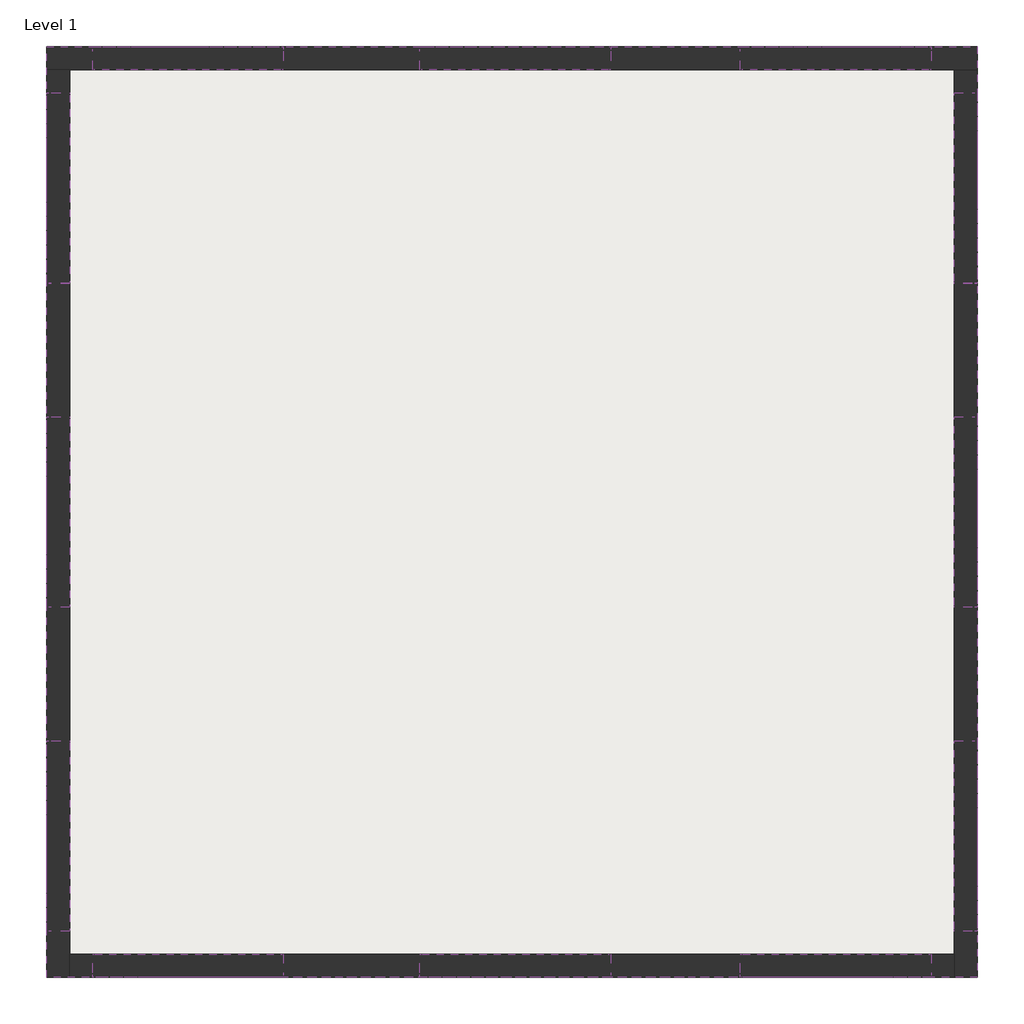
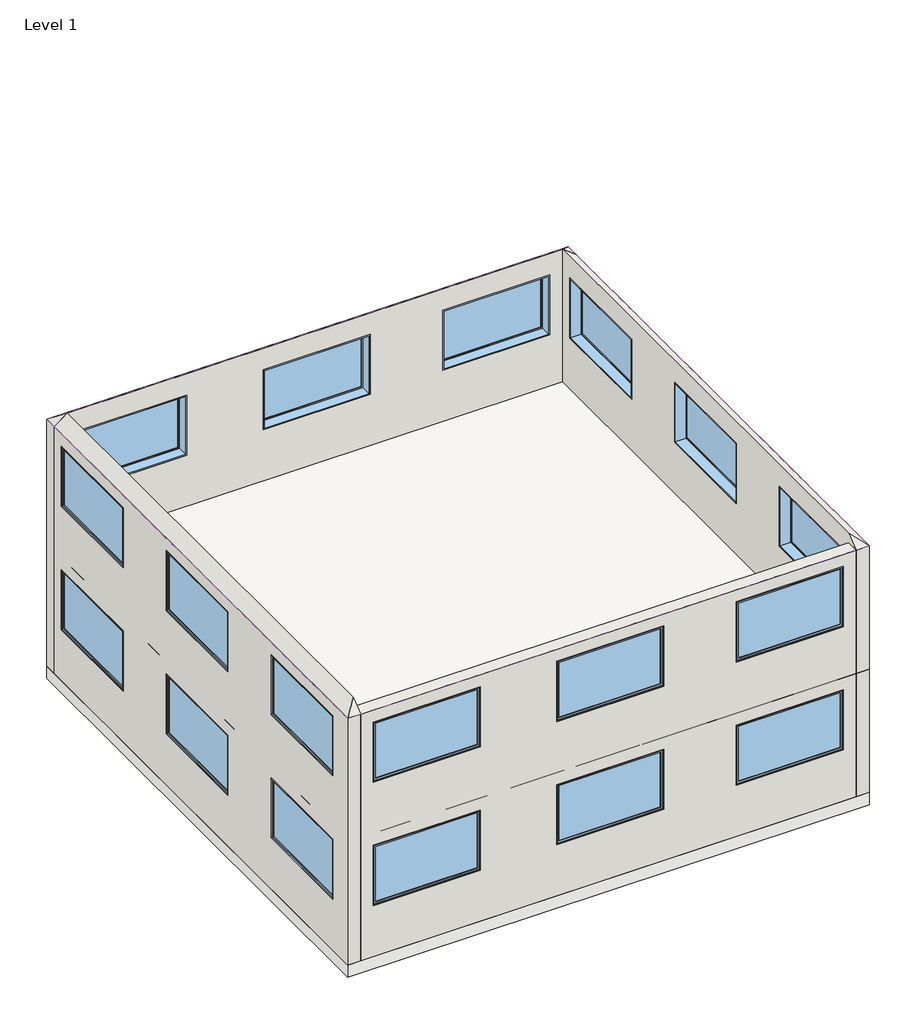
# One storey: 24 windows, 4 walls, 2 slabs, 1 roof.
"""IFC4 building model written with IfcOpenShell, lengths in millimetres."""

import ifcopenshell
import ifcopenshell.guid

model = None  # the IFC model being written
_history = None  # IfcOwnerHistory: only IFC2X3 demands one
_inside = {}  # id of a spatial element -> (the spatial element, [elements in it])
_under = {}  # id of a project, library or spatial element -> (it, [spatial elements below it])
_declared = {}  # id of a project -> (the project, [libraries it declares])
_typed = {}  # id of a type object -> (the type object, [elements of that type])
_made_of = {}  # id of a material, layer set ... -> (it, [elements and type objects made of it])


def new_model(schema):
    """Start an empty IFC model of exactly this schema.

    Asked for "IFC4X3", IfcOpenShell would pick the latest addendum, in which some entities
    have other attributes; the version numbers below select the first issue.
    IFC2X3 requires an IfcOwnerHistory on every rooted entity: one is made here for all.
    """
    global model, _history
    if schema == "IFC4X3":
        model = ifcopenshell.file(schema_version=(4, 3, 0, 0))
    else:
        model = ifcopenshell.file(schema=schema)
    _inside.clear()
    _under.clear()
    _declared.clear()
    _typed.clear()
    _made_of.clear()
    _history = None
    if model.schema == "IFC2X3":
        org = make("IfcOrganization", Name="unknown")
        user = make(
            "IfcPersonAndOrganization",
            ThePerson=make("IfcPerson", FamilyName="unknown"),
            TheOrganization=org,
        )
        app = make(
            "IfcApplication",
            ApplicationDeveloper=org,
            Version="unknown",
            ApplicationFullName="unknown",
            ApplicationIdentifier="unknown",
        )
        _history = make(
            "IfcOwnerHistory",
            OwningUser=user,
            OwningApplication=app,
            ChangeAction="ADDED",
            CreationDate=0,
        )
    return model


def make(cls, **values):
    """One entity of the class cls with the attributes given. An attribute that is None is left unset."""
    return model.create_entity(
        cls, **{name: value for name, value in values.items() if value is not None}
    )


def rooted(cls, **values):
    """An entity with a GlobalId (a new one), such as an element, a storey or a relation."""
    return make(cls, GlobalId=ifcopenshell.guid.new(), OwnerHistory=_history, **values)


def si_unit(unit_type, name, prefix=None):
    """IfcSIUnit, for example si_unit("LENGTHUNIT", "METRE", prefix="MILLI")."""
    return make("IfcSIUnit", UnitType=unit_type, Prefix=prefix, Name=name)


def assignment(units):
    """IfcUnitAssignment: the units of a project."""
    return None if units is None else make("IfcUnitAssignment", Units=units)


def point(xyz):
    """IfcCartesianPoint."""
    return None if xyz is None else make("IfcCartesianPoint", Coordinates=xyz)


def direction(xyz):
    """IfcDirection."""
    return None if xyz is None else make("IfcDirection", DirectionRatios=xyz)


def frame(location, z_axis=None, x_axis=None):
    """IfcAxis2Placement3D, a coordinate frame: its origin and axes. An axis left out is left unset."""
    return make(
        "IfcAxis2Placement3D",
        Location=point(location),
        Axis=direction(z_axis),
        RefDirection=direction(x_axis),
    )


def origin():
    """The frame at (0, 0, 0) with its axes left unset."""
    return frame((0.0, 0.0, 0.0))


def place(relative_to, where):
    """IfcLocalPlacement: puts the frame where relative to a parent placement (None: the world)."""
    return make(
        "IfcLocalPlacement", PlacementRelTo=relative_to, RelativePlacement=where
    )


def context(
    kind, dimensions, precision=None, world=None, true_north=None, identifier=None
):
    """IfcGeometricRepresentationContext, for example the 3D "Model" context."""
    return make(
        "IfcGeometricRepresentationContext",
        ContextIdentifier=identifier,
        ContextType=kind,
        CoordinateSpaceDimension=dimensions,
        Precision=precision,
        WorldCoordinateSystem=world,
        TrueNorth=true_north,
    )


def project(units=None, contexts=None):
    """IfcProject with its units and contexts."""
    return rooted(
        "IfcProject",
        Name="project",
        RepresentationContexts=contexts,
        UnitsInContext=assignment(units),
    )


def spatial(cls, under=None, at=None, **own):
    """A site, building, storey or space (cls), placed at a placement, below another one or the project."""
    s = rooted(cls, ObjectPlacement=at, **own)
    if under is not None:
        _under.setdefault(under.id(), (under, []))[1].append(s)
    return s


def polyline(points):
    """IfcPolyline through the points."""
    return make("IfcPolyline", Points=[point(p) for p in points])


def outline(outer, holes=None, kind="AREA"):
    """IfcArbitraryClosedProfileDef: a profile drawn as a closed curve; with holes, ...WithVoids."""
    if holes is None:
        return make("IfcArbitraryClosedProfileDef", ProfileType=kind, OuterCurve=outer)
    return make(
        "IfcArbitraryProfileDefWithVoids",
        ProfileType=kind,
        OuterCurve=outer,
        InnerCurves=holes,
    )


def extrude(swept, where, along, depth):
    """IfcExtrudedAreaSolid: the profile swept, set in the frame where, extruded along a direction by depth."""
    return make(
        "IfcExtrudedAreaSolid",
        SweptArea=swept,
        Position=where,
        ExtrudedDirection=direction(along),
        Depth=depth,
    )


def faces_of(points, faces, orient=None, outer=None):
    """IfcFace entities. A face is a list of loops; a loop is a list of indices into points, from 0.

    orient and outer hold one flag for each loop. By default every Orientation is true, the
    first loop of a face is its IfcFaceOuterBound and the others are IfcFaceBound.
    """
    made = []
    for i, loops in enumerate(faces):
        bounds = []
        for j, loop in enumerate(loops):
            is_outer = j == 0 if outer is None else outer[i][j]
            bounds.append(
                make(
                    "IfcFaceOuterBound" if is_outer else "IfcFaceBound",
                    Bound=make("IfcPolyLoop", Polygon=[points[k] for k in loop]),
                    Orientation=True if orient is None else orient[i][j],
                )
            )
        made.append(make("IfcFace", Bounds=bounds))
    return made


def faceted_brep(points, faces, orient=None, outer=None, voids=None):
    """IfcFacetedBrep: a solid bounded by flat faces; with voids (closed shells), ...WithVoids."""
    shared = [point(p) for p in points]
    hull = make("IfcClosedShell", CfsFaces=faces_of(shared, faces, orient, outer))
    if voids is None:
        return make("IfcFacetedBrep", Outer=hull)
    return make(
        "IfcFacetedBrepWithVoids",
        Outer=hull,
        Voids=[
            make(cls, CfsFaces=faces_of(shared, fs, o, b)) for cls, fs, o, b in voids
        ],
    )


def shape(context_of_items, identifier, shape_type, items):
    """IfcShapeRepresentation: the items that make up one representation, for example the "Body"."""
    return make(
        "IfcShapeRepresentation",
        ContextOfItems=context_of_items,
        RepresentationIdentifier=identifier,
        RepresentationType=shape_type,
        Items=items,
    )


def source(mapping_origin, context_of_items, identifier, shape_type, items):
    """IfcRepresentationMap: a shape defined once, which mapped items show again and again."""
    return make(
        "IfcRepresentationMap",
        MappingOrigin=mapping_origin,
        MappedRepresentation=shape(context_of_items, identifier, shape_type, items),
    )


def transform(
    local_origin,
    x_axis=None,
    y_axis=None,
    z_axis=None,
    scale=None,
    scale2=None,
    scale3=None,
    uniform=True,
):
    """IfcCartesianTransformationOperator3D, or its non-uniform kind. x_axis, y_axis, z_axis: its Axis1, 2, 3."""
    if uniform:
        return make(
            "IfcCartesianTransformationOperator3D",
            Axis1=direction(x_axis),
            Axis2=direction(y_axis),
            LocalOrigin=point(local_origin),
            Scale=scale,
            Axis3=direction(z_axis),
        )
    return make(
        "IfcCartesianTransformationOperator3DnonUniform",
        Axis1=direction(x_axis),
        Axis2=direction(y_axis),
        LocalOrigin=point(local_origin),
        Scale=scale,
        Axis3=direction(z_axis),
        Scale2=scale2,
        Scale3=scale3,
    )


def mapped(mapping_source, mapping_target):
    """IfcMappedItem: shows the shape of a source again, moved by a transform."""
    return make(
        "IfcMappedItem", MappingSource=mapping_source, MappingTarget=mapping_target
    )


def made_of(thing, what):
    """Note that an element or type object is made of a material, layer set ...; save() writes the relation."""
    if what is not None:
        _made_of.setdefault(what.id(), (what, []))[1].append(thing)
    return thing


def element(
    cls,
    number,
    at=None,
    inside=None,
    cuts=None,
    type_object=None,
    material=None,
    context=None,
    identifier="Body",
    shape_type=None,
    held_by="IfcProductDefinitionShape",
    body=None,
    shapes=None,
    **own,
):
    """One element of the class cls, such as IfcWall. Its Tag is "e" and its number.

    at: its placement. inside: the storey or other place that contains it. cuts: it is an
    opening in that element (IfcRelVoidsElement). A single representation is given by context,
    identifier, shape_type and body (its items); several are given by shapes. held_by: the class
    of the entity that holds the representations. save() writes the other relations.
    """
    e = rooted(cls, Tag="e%d" % number, ObjectPlacement=at, **own)
    if body is not None:
        shapes = [shape(context, identifier, shape_type, body)]
    if shapes is not None:
        e.Representation = make(held_by, Representations=shapes)
    if inside is not None:
        _inside.setdefault(inside.id(), (inside, []))[1].append(e)
    if cuts is not None:
        rooted(
            "IfcRelVoidsElement", RelatingBuildingElement=cuts, RelatedOpeningElement=e
        )
    if type_object is not None:
        _typed.setdefault(type_object.id(), (type_object, []))[1].append(e)
    return made_of(e, material)


def aggregate(whole, parts):
    """IfcRelAggregates: a whole, such as a stair, and the parts it consists of."""
    return rooted("IfcRelAggregates", RelatingObject=whole, RelatedObjects=parts)


def save(model, path):
    """Write the relations noted so far, then the file.

    IfcRelAggregates (storeys below a building ...), IfcRelContainedInSpatialStructure (elements
    in a storey), IfcRelDefinesByType, IfcRelAssociatesMaterial and IfcRelDeclares: one each for
    every whole, place, type object, material and project.
    """
    for whole, parts in _under.values():
        aggregate(whole, parts)
    for where, things in _inside.values():
        rooted(
            "IfcRelContainedInSpatialStructure",
            RelatedElements=things,
            RelatingStructure=where,
        )
    for kind, things in _typed.values():
        rooted("IfcRelDefinesByType", RelatedObjects=things, RelatingType=kind)
    for what, things in _made_of.values():
        rooted("IfcRelAssociatesMaterial", RelatedObjects=things, RelatingMaterial=what)
    for by, libraries in _declared.values():
        rooted("IfcRelDeclares", RelatingContext=by, RelatedDefinitions=libraries)
    model.write(path)


def m_fixed_2500_x_1486mm_baf7df51(model_context):
    return source(origin(), model_context, "Body", "SweptSolid", [
        extrude(outline(polyline([(-1187.0, 130.4), (1187.0, 130.4), (1187.0, 118.4), (-1187.0, 118.4), (-1187.0, 130.4)])), frame((0.0, 0.0, 978.0), z_axis=(0.0, 0.0, 1.0), x_axis=(1.0, 0.0, 0.0)), (0.0, 0.0, 1.0), 1360.5),
        extrude(outline(polyline([(2382.5, -1231.0), (934.0, -1231.0), (934.0, 1231.0), (2382.5, 1231.0), (2382.5, -1231.0)]), holes=[polyline([(2338.5, -1187.0), (2338.5, 1187.0), (978.0, 1187.0), (978.0, -1187.0), (2338.5, -1187.0)])]), frame((0.0, 102.4, 0.0), z_axis=(0.0, 1.0, 0.0), x_axis=(0.0, 0.0, 1.0)), (0.0, 0.0, 1.0), 44.0),
        extrude(outline(polyline([(2401.5, -1250.0), (915.0, -1250.0), (915.0, 1250.0), (2401.5, 1250.0), (2401.5, -1250.0)]), holes=[polyline([(2382.5, -1231.0), (2382.5, 1231.0), (934.0, 1231.0), (934.0, -1231.0), (2382.5, -1231.0)])]), frame((0.0, 102.4, 0.0), z_axis=(0.0, 1.0, 0.0), x_axis=(0.0, 0.0, 1.0)), (0.0, 0.0, 1.0), 63.0),
        extrude(outline(polyline([(2401.5, -1250.0), (915.0, -1250.0), (915.0, 1250.0), (2401.5, 1250.0), (2401.5, -1250.0)]), holes=[polyline([(2369.5, -1218.0), (2369.5, 1218.0), (947.0, 1218.0), (947.0, -1218.0), (2369.5, -1218.0)])]), frame((0.0, -139.4, 0.0), z_axis=(0.0, 1.0, 0.0), x_axis=(0.0, 0.0, 1.0)), (0.0, 0.0, 1.0), 241.8),
    ])


def m_fixed_2500_x_1486mm_49bc14c1(model_context):
    return source(origin(), model_context, "Body", "SweptSolid", [
        extrude(outline(polyline([(-1187.0, -130.4), (-1187.0, -118.4), (1187.0, -118.4), (1187.0, -130.4), (-1187.0, -130.4)])), frame((0.0, 0.0, 978.0), z_axis=(0.0, 0.0, 1.0), x_axis=(1.0, 0.0, 0.0)), (0.0, 0.0, 1.0), 1360.5),
        extrude(outline(polyline([(2382.5, -1231.0), (934.0, -1231.0), (934.0, 1231.0), (2382.5, 1231.0), (2382.5, -1231.0)]), holes=[polyline([(2338.5, -1187.0), (2338.5, 1187.0), (978.0, 1187.0), (978.0, -1187.0), (2338.5, -1187.0)])]), frame((0.0, -146.4, 0.0), z_axis=(0.0, 1.0, 0.0), x_axis=(0.0, 0.0, 1.0)), (0.0, 0.0, 1.0), 44.0),
        extrude(outline(polyline([(2401.5, -1250.0), (915.0, -1250.0), (915.0, 1250.0), (2401.5, 1250.0), (2401.5, -1250.0)]), holes=[polyline([(2382.5, -1231.0), (2382.5, 1231.0), (934.0, 1231.0), (934.0, -1231.0), (2382.5, -1231.0)])]), frame((0.0, -165.4, 0.0), z_axis=(0.0, 1.0, 0.0), x_axis=(0.0, 0.0, 1.0)), (0.0, 0.0, 1.0), 63.0),
        extrude(outline(polyline([(2401.5, -1250.0), (915.0, -1250.0), (915.0, 1250.0), (2401.5, 1250.0), (2401.5, -1250.0)]), holes=[polyline([(2369.5, -1218.0), (2369.5, 1218.0), (947.0, 1218.0), (947.0, -1218.0), (2369.5, -1218.0)])]), frame((0.0, -102.4, 0.0), z_axis=(0.0, 1.0, 0.0), x_axis=(0.0, 0.0, 1.0)), (0.0, 0.0, 1.0), 241.8),
    ])


model = new_model("IFC4")

# Units and contexts
model_context = context("Model", 3, world=origin())
ifc_project = project(units=[si_unit("LENGTHUNIT", "METRE", prefix="MILLI")], contexts=[model_context])

# Site, building, storey
site = spatial("IfcSite", under=ifc_project)
building = spatial("IfcBuilding", under=site)
storey = spatial("IfcBuildingStorey", under=building, Name="Level 1", Elevation=0.0)

# Roof
placement = place(None, origin())
element("IfcRoof", 1, ObjectType="Generic Roof - 300mm", at=placement, inside=storey, context=model_context, shape_type="Brep", body=[
    faceted_brep([(21465.644102, 9062.7173115, 6096.0), (15369.644102, 2966.7173115, 10668.0170156), (9273.644102, 9062.7173115, 6096.0), (9273.644102, -3129.2826885, 6096.0), (13109.1679245, -3129.2826885, 6096.0), (12998.044102, -3129.2826885, 6096.0), (21465.644102, -3129.2826885, 6096.0), (17741.244102, -3129.2826885, 6096.0), (17630.1202795, -3129.2826885, 6096.0), (15369.644102, 1410.2073073, 9500.6301678), (15369.644102, -3129.2826885, 9500.6301678), (21465.644102, 9062.7173115, 6471.0005024), (9273.644102, 9062.7173115, 6471.0005024), (15369.644102, 2966.7173115, 11043.0175181), (9273.644102, -3129.2826885, 6471.0005024), (12998.044102, -3129.2826885, 6471.0005024), (15369.644102, 1633.366253, 10043.0005024), (17741.244102, -3129.2826885, 6471.0005024), (21465.644102, -3129.2826885, 6471.0005024), (15369.644102, -3129.2826885, 10043.0005024)], [[[0, 1, 2]], [[2, 1, 3]], [[4, 5, 3, 1, 6, 7, 8, 9]], [[6, 1, 0]], [[4, 9, 10]], [[8, 10, 9]], [[11, 12, 13]], [[12, 14, 13]], [[15, 16, 17, 18, 13, 14]], [[18, 11, 13]], [[15, 19, 16]], [[17, 16, 19]], [[6, 18, 17, 7]], [[0, 11, 18, 6]], [[2, 12, 11, 0]], [[3, 14, 12, 2]], [[5, 15, 14, 3]], [[17, 19, 15, 5, 4, 10, 8, 7]]]),
])

# Slabs
element("IfcSlab", 2, ObjectType="Generic Floor - 304.8mm", at=placement, inside=storey, context=model_context, shape_type="Brep", body=[
    faceted_brep([(21465.644102, 9062.7173115, -304.8), (21465.644102, -3129.2826885, -304.8), (9273.644102, -3129.2826885, -304.8), (9273.644102, 9062.7173115, -304.8), (21465.644102, 9062.7173115, 0.0), (9273.644102, 9062.7173115, 0.0), (9273.644102, -3129.2826885, 0.0), (9578.444102, -3129.2826885, 0.0), (21160.844102, -3129.2826885, 0.0), (21465.644102, -3129.2826885, 0.0), (21465.644102, 8757.9173115, 0.0)], [[[0, 1, 2, 3]], [[4, 5, 6, 7, 8, 9, 10]], [[1, 0, 4, 10, 9]], [[2, 1, 9, 8, 7, 6]], [[3, 2, 6, 5]], [[0, 3, 5, 4]]]),
])
element("IfcSlab", 3, ObjectType="Generic Floor - 304.8mm", at=placement, inside=storey, context=model_context, shape_type="SweptSolid", body=[
    extrude(outline(polyline([(21465.644102, 9062.7173115), (21465.644102, -3129.2826885), (9273.644102, -3129.2826885), (9273.644102, 9062.7173115), (21465.644102, 9062.7173115)])), frame((0.0, 0.0, 2743.2), z_axis=(0.0, 0.0, 1.0), x_axis=(1.0, 0.0, 0.0)), (0.0, 0.0, 1.0), 304.8),
])

# Walls
element("IfcWall", 4, ObjectType="Generic - 304.8mm", at=placement, inside=storey, context=model_context, shape_type="Brep", body=[
    faceted_brep([(9273.644102, 8757.9173115, 0.0), (9578.444102, 8757.9173115, 0.0), (21160.844102, 8757.9173115, 0.0), (21465.644102, 8757.9173115, 0.0), (21465.644102, 8757.9173115, 6096.0), (21160.844102, 8757.9173115, 6324.6008508), (9578.444102, 8757.9173115, 6324.6008508), (9273.644102, 8757.9173115, 6096.0), (14163.244102, 8757.9173115, 4309.5), (14163.244102, 8757.9173115, 5796.0), (16663.244102, 8757.9173115, 5796.0), (16663.244102, 8757.9173115, 4309.5), (9876.044102, 8757.9173115, 4309.5), (9876.044102, 8757.9173115, 5796.0), (12376.044102, 8757.9173115, 5796.0), (12376.044102, 8757.9173115, 4309.5), (18363.244102, 8757.9173115, 4309.5), (18363.244102, 8757.9173115, 5796.0), (20863.244102, 8757.9173115, 5796.0), (20863.244102, 8757.9173115, 4309.5), (18363.244102, 8757.9173115, 1261.5), (18363.244102, 8757.9173115, 2748.0), (20863.244102, 8757.9173115, 2748.0), (20863.244102, 8757.9173115, 1261.5), (9876.044102, 8757.9173115, 1261.5), (9876.044102, 8757.9173115, 2748.0), (12376.044102, 8757.9173115, 2748.0), (12376.044102, 8757.9173115, 1261.5), (14163.244102, 8757.9173115, 1261.5), (14163.244102, 8757.9173115, 2748.0), (16663.244102, 8757.9173115, 2748.0), (16663.244102, 8757.9173115, 1261.5), (9273.644102, 9062.7173115, 0.0), (9273.644102, 9062.7173115, 6096.0), (21465.644102, 9062.7173115, 6096.0), (21465.644102, 9062.7173115, 0.0), (14163.244102, 9062.7173115, 4309.5), (16663.244102, 9062.7173115, 4309.5), (16663.244102, 9062.7173115, 5796.0), (14163.244102, 9062.7173115, 5796.0), (9876.044102, 9062.7173115, 4309.5), (12376.044102, 9062.7173115, 4309.5), (12376.044102, 9062.7173115, 5796.0), (9876.044102, 9062.7173115, 5796.0), (18363.244102, 9062.7173115, 4309.5), (20863.244102, 9062.7173115, 4309.5), (20863.244102, 9062.7173115, 5796.0), (18363.244102, 9062.7173115, 5796.0), (18363.244102, 9062.7173115, 1261.5), (20863.244102, 9062.7173115, 1261.5), (20863.244102, 9062.7173115, 2748.0), (18363.244102, 9062.7173115, 2748.0), (9876.044102, 9062.7173115, 1261.5), (12376.044102, 9062.7173115, 1261.5), (12376.044102, 9062.7173115, 2748.0), (9876.044102, 9062.7173115, 2748.0), (14163.244102, 9062.7173115, 1261.5), (16663.244102, 9062.7173115, 1261.5), (16663.244102, 9062.7173115, 2748.0), (14163.244102, 9062.7173115, 2748.0)], [[[0, 1, 2, 3, 4, 5, 6, 7], [8, 9, 10, 11], [12, 13, 14, 15], [16, 17, 18, 19], [20, 21, 22, 23], [24, 25, 26, 27], [28, 29, 30, 31]], [[32, 33, 34, 35], [36, 37, 38, 39], [40, 41, 42, 43], [44, 45, 46, 47], [48, 49, 50, 51], [52, 53, 54, 55], [56, 57, 58, 59]], [[3, 2, 1, 0, 32, 35]], [[4, 3, 35, 34]], [[0, 7, 33, 32]], [[9, 8, 36, 39]], [[10, 9, 39, 38]], [[11, 10, 38, 37]], [[8, 11, 37, 36]], [[13, 12, 40, 43]], [[14, 13, 43, 42]], [[15, 14, 42, 41]], [[12, 15, 41, 40]], [[17, 16, 44, 47]], [[18, 17, 47, 46]], [[19, 18, 46, 45]], [[16, 19, 45, 44]], [[21, 20, 48, 51]], [[22, 21, 51, 50]], [[23, 22, 50, 49]], [[20, 23, 49, 48]], [[25, 24, 52, 55]], [[26, 25, 55, 54]], [[27, 26, 54, 53]], [[24, 27, 53, 52]], [[29, 28, 56, 59]], [[30, 29, 59, 58]], [[31, 30, 58, 57]], [[28, 31, 57, 56]], [[7, 6, 33]], [[6, 5, 34, 33]], [[5, 4, 34]]]),
])
element("IfcWall", 5, ObjectType="Generic - 304.8mm", at=placement, inside=storey, context=model_context, shape_type="Brep", body=[
    faceted_brep([(21160.844102, 8757.9173115, 0.0), (21160.844102, -2824.4826885, 0.0), (21160.844102, -3129.2826885, 0.0), (21160.844102, -3129.2826885, 6096.0), (21160.844102, -2824.4826885, 6324.6008508), (21160.844102, 8757.9173115, 6324.6008508), (21160.844102, -26.8826885, 4309.5), (21160.844102, -26.8826885, 5796.0), (21160.844102, -2526.8826885, 5796.0), (21160.844102, -2526.8826885, 4309.5), (21160.844102, 8460.3173115, 4309.5), (21160.844102, 8460.3173115, 5796.0), (21160.844102, 5960.3173115, 5796.0), (21160.844102, 5960.3173115, 4309.5), (21160.844102, 4216.7173115, 4309.5), (21160.844102, 4216.7173115, 5796.0), (21160.844102, 1716.7173115, 5796.0), (21160.844102, 1716.7173115, 4309.5), (21160.844102, 4216.7173115, 1261.5), (21160.844102, 4216.7173115, 2748.0), (21160.844102, 1716.7173115, 2748.0), (21160.844102, 1716.7173115, 1261.5), (21160.844102, 8460.3173115, 1261.5), (21160.844102, 8460.3173115, 2748.0), (21160.844102, 5960.3173115, 2748.0), (21160.844102, 5960.3173115, 1261.5), (21160.844102, -26.8826885, 1261.5), (21160.844102, -26.8826885, 2748.0), (21160.844102, -2526.8826885, 2748.0), (21160.844102, -2526.8826885, 1261.5), (21465.644102, 8757.9173115, 0.0), (21465.644102, 8757.9173115, 6096.0), (21465.644102, -3129.2826885, 6096.0), (21465.644102, -3129.2826885, 0.0), (21465.644102, -26.8826885, 4309.5), (21465.644102, -2526.8826885, 4309.5), (21465.644102, -2526.8826885, 5796.0), (21465.644102, -26.8826885, 5796.0), (21465.644102, 8460.3173115, 4309.5), (21465.644102, 5960.3173115, 4309.5), (21465.644102, 5960.3173115, 5796.0), (21465.644102, 8460.3173115, 5796.0), (21465.644102, 4216.7173115, 4309.5), (21465.644102, 1716.7173115, 4309.5), (21465.644102, 1716.7173115, 5796.0), (21465.644102, 4216.7173115, 5796.0), (21465.644102, 4216.7173115, 1261.5), (21465.644102, 1716.7173115, 1261.5), (21465.644102, 1716.7173115, 2748.0), (21465.644102, 4216.7173115, 2748.0), (21465.644102, 8460.3173115, 1261.5), (21465.644102, 5960.3173115, 1261.5), (21465.644102, 5960.3173115, 2748.0), (21465.644102, 8460.3173115, 2748.0), (21465.644102, -26.8826885, 1261.5), (21465.644102, -2526.8826885, 1261.5), (21465.644102, -2526.8826885, 2748.0), (21465.644102, -26.8826885, 2748.0)], [[[0, 1, 2, 3, 4, 5], [6, 7, 8, 9], [10, 11, 12, 13], [14, 15, 16, 17], [18, 19, 20, 21], [22, 23, 24, 25], [26, 27, 28, 29]], [[30, 31, 32, 33], [34, 35, 36, 37], [38, 39, 40, 41], [42, 43, 44, 45], [46, 47, 48, 49], [50, 51, 52, 53], [54, 55, 56, 57]], [[2, 1, 0, 30, 33]], [[0, 5, 31, 30]], [[3, 2, 33, 32]], [[7, 6, 34, 37]], [[8, 7, 37, 36]], [[9, 8, 36, 35]], [[6, 9, 35, 34]], [[11, 10, 38, 41]], [[12, 11, 41, 40]], [[13, 12, 40, 39]], [[10, 13, 39, 38]], [[15, 14, 42, 45]], [[16, 15, 45, 44]], [[17, 16, 44, 43]], [[14, 17, 43, 42]], [[19, 18, 46, 49]], [[20, 19, 49, 48]], [[21, 20, 48, 47]], [[18, 21, 47, 46]], [[23, 22, 50, 53]], [[24, 23, 53, 52]], [[25, 24, 52, 51]], [[22, 25, 51, 50]], [[27, 26, 54, 57]], [[28, 27, 57, 56]], [[29, 28, 56, 55]], [[26, 29, 55, 54]], [[5, 4, 32, 31]], [[4, 3, 32]]]),
])
element("IfcWall", 6, ObjectType="Generic - 304.8mm", at=placement, inside=storey, context=model_context, shape_type="Brep", body=[
    faceted_brep([(9578.444102, -3129.2826885, 0.0), (9578.444102, -2824.4826885, 0.0), (9578.444102, 8757.9173115, 0.0), (9578.444102, 8757.9173115, 6324.6008508), (9578.444102, -2824.4826885, 6324.6008508), (9578.444102, -3129.2826885, 6096.0), (9578.444102, 1716.7173115, 4309.5), (9578.444102, 1716.7173115, 5796.0), (9578.444102, 4216.7173115, 5796.0), (9578.444102, 4216.7173115, 4309.5), (9578.444102, 5960.3173115, 4309.5), (9578.444102, 5960.3173115, 5796.0), (9578.444102, 8460.3173115, 5796.0), (9578.444102, 8460.3173115, 4309.5), (9578.444102, -2526.8826885, 4309.5), (9578.444102, -2526.8826885, 5796.0), (9578.444102, -26.8826885, 5796.0), (9578.444102, -26.8826885, 4309.5), (9578.444102, -2526.8826885, 1261.5), (9578.444102, -2526.8826885, 2748.0), (9578.444102, -26.8826885, 2748.0), (9578.444102, -26.8826885, 1261.5), (9578.444102, 5960.3173115, 1261.5), (9578.444102, 5960.3173115, 2748.0), (9578.444102, 8460.3173115, 2748.0), (9578.444102, 8460.3173115, 1261.5), (9578.444102, 1716.7173115, 1261.5), (9578.444102, 1716.7173115, 2748.0), (9578.444102, 4216.7173115, 2748.0), (9578.444102, 4216.7173115, 1261.5), (9273.644102, -3129.2826885, 0.0), (9273.644102, -3129.2826885, 6096.0), (9273.644102, 8757.9173115, 6096.0), (9273.644102, 8757.9173115, 0.0), (9273.644102, 1716.7173115, 4309.5), (9273.644102, 4216.7173115, 4309.5), (9273.644102, 4216.7173115, 5796.0), (9273.644102, 1716.7173115, 5796.0), (9273.644102, 5960.3173115, 4309.5), (9273.644102, 8460.3173115, 4309.5), (9273.644102, 8460.3173115, 5796.0), (9273.644102, 5960.3173115, 5796.0), (9273.644102, -2526.8826885, 4309.5), (9273.644102, -26.8826885, 4309.5), (9273.644102, -26.8826885, 5796.0), (9273.644102, -2526.8826885, 5796.0), (9273.644102, -2526.8826885, 1261.5), (9273.644102, -26.8826885, 1261.5), (9273.644102, -26.8826885, 2748.0), (9273.644102, -2526.8826885, 2748.0), (9273.644102, 5960.3173115, 1261.5), (9273.644102, 8460.3173115, 1261.5), (9273.644102, 8460.3173115, 2748.0), (9273.644102, 5960.3173115, 2748.0), (9273.644102, 1716.7173115, 1261.5), (9273.644102, 4216.7173115, 1261.5), (9273.644102, 4216.7173115, 2748.0), (9273.644102, 1716.7173115, 2748.0)], [[[0, 1, 2, 3, 4, 5], [6, 7, 8, 9], [10, 11, 12, 13], [14, 15, 16, 17], [18, 19, 20, 21], [22, 23, 24, 25], [26, 27, 28, 29]], [[30, 31, 32, 33], [34, 35, 36, 37], [38, 39, 40, 41], [42, 43, 44, 45], [46, 47, 48, 49], [50, 51, 52, 53], [54, 55, 56, 57]], [[2, 1, 0, 30, 33]], [[3, 2, 33, 32]], [[0, 5, 31, 30]], [[7, 6, 34, 37]], [[8, 7, 37, 36]], [[9, 8, 36, 35]], [[6, 9, 35, 34]], [[11, 10, 38, 41]], [[12, 11, 41, 40]], [[13, 12, 40, 39]], [[10, 13, 39, 38]], [[15, 14, 42, 45]], [[16, 15, 45, 44]], [[17, 16, 44, 43]], [[14, 17, 43, 42]], [[19, 18, 46, 49]], [[20, 19, 49, 48]], [[21, 20, 48, 47]], [[18, 21, 47, 46]], [[23, 22, 50, 53]], [[24, 23, 53, 52]], [[25, 24, 52, 51]], [[22, 25, 51, 50]], [[27, 26, 54, 57]], [[28, 27, 57, 56]], [[29, 28, 56, 55]], [[26, 29, 55, 54]], [[5, 4, 31]], [[4, 3, 32, 31]]]),
])
element("IfcWall", 7, ObjectType="Generic - 304.8mm", at=placement, inside=storey, context=model_context, shape_type="SweptSolid", body=[
    extrude(outline(polyline([(0.0, 9578.444102), (0.0, 21160.844102), (6096.0, 21160.844102), (6096.0, 9578.444102), (0.0, 9578.444102)]), holes=[polyline([(4309.5, 14163.244102), (5796.0, 14163.244102), (5796.0, 16663.244102), (4309.5, 16663.244102), (4309.5, 14163.244102)]), polyline([(4309.5, 9876.044102), (5796.0, 9876.044102), (5796.0, 12376.044102), (4309.5, 12376.044102), (4309.5, 9876.044102)]), polyline([(4309.5, 18363.244102), (5796.0, 18363.244102), (5796.0, 20863.244102), (4309.5, 20863.244102), (4309.5, 18363.244102)]), polyline([(1261.5, 18363.244102), (2748.0, 18363.244102), (2748.0, 20863.244102), (1261.5, 20863.244102), (1261.5, 18363.244102)]), polyline([(1261.5, 9876.044102), (2748.0, 9876.044102), (2748.0, 12376.044102), (1261.5, 12376.044102), (1261.5, 9876.044102)]), polyline([(1261.5, 14163.244102), (2748.0, 14163.244102), (2748.0, 16663.244102), (1261.5, 16663.244102), (1261.5, 14163.244102)])]), frame((0.0, -3129.2826885, 0.0), z_axis=(0.0, 1.0, 0.0), x_axis=(0.0, 0.0, 1.0)), (0.0, 0.0, 1.0), 304.8),
])

# Windows
m_fixed_2500_x_1486mm_shape = m_fixed_2500_x_1486mm_baf7df51(model_context)
element("IfcWindow", 8, ObjectType="M_Fixed : 2500 x 1486mm", at=placement, inside=storey, context=model_context, shape_type="MappedRepresentation", body=[
    mapped(m_fixed_2500_x_1486mm_shape, transform((15413.244102, 8897.3173115, 3394.5), x_axis=(1.0, 0.0, 0.0), y_axis=(0.0, 1.0, 0.0), z_axis=(0.0, 0.0, 1.0))),
])
element("IfcWindow", 9, ObjectType="M_Fixed : 2500 x 1486mm", at=placement, inside=storey, context=model_context, shape_type="MappedRepresentation", body=[
    mapped(m_fixed_2500_x_1486mm_shape, transform((11126.044102, 8897.3173115, 3394.5), x_axis=(1.0, 0.0, 0.0), y_axis=(0.0, 1.0, 0.0), z_axis=(0.0, 0.0, 1.0))),
])
element("IfcWindow", 10, ObjectType="M_Fixed : 2500 x 1486mm", at=placement, inside=storey, context=model_context, shape_type="MappedRepresentation", body=[
    mapped(m_fixed_2500_x_1486mm_shape, transform((19613.244102, 8897.3173115, 3394.5), x_axis=(1.0, 0.0, 0.0), y_axis=(0.0, 1.0, 0.0), z_axis=(0.0, 0.0, 1.0))),
])
element("IfcWindow", 11, ObjectType="M_Fixed : 2500 x 1486mm", at=placement, inside=storey, context=model_context, shape_type="MappedRepresentation", body=[
    mapped(m_fixed_2500_x_1486mm_shape, transform((15413.244102, 8897.3173115, 346.5), x_axis=(1.0, 0.0, 0.0), y_axis=(0.0, 1.0, 0.0), z_axis=(0.0, 0.0, 1.0))),
])
element("IfcWindow", 12, ObjectType="M_Fixed : 2500 x 1486mm", at=placement, inside=storey, context=model_context, shape_type="MappedRepresentation", body=[
    mapped(m_fixed_2500_x_1486mm_shape, transform((11126.044102, 8897.3173115, 346.5), x_axis=(1.0, 0.0, 0.0), y_axis=(0.0, 1.0, 0.0), z_axis=(0.0, 0.0, 1.0))),
])
element("IfcWindow", 13, ObjectType="M_Fixed : 2500 x 1486mm", at=placement, inside=storey, context=model_context, shape_type="MappedRepresentation", body=[
    mapped(m_fixed_2500_x_1486mm_shape, transform((19613.244102, 8897.3173115, 346.5), x_axis=(1.0, 0.0, 0.0), y_axis=(0.0, 1.0, 0.0), z_axis=(0.0, 0.0, 1.0))),
])
element("IfcWindow", 14, ObjectType="M_Fixed : 2500 x 1486mm", at=placement, inside=storey, context=model_context, shape_type="MappedRepresentation", body=[
    mapped(m_fixed_2500_x_1486mm_shape, transform((21300.244102, -1276.8826885, 3394.5), x_axis=(0.0, -1.0, 0.0), y_axis=(1.0, 0.0, 0.0), z_axis=(0.0, 0.0, 1.0))),
])
element("IfcWindow", 15, ObjectType="M_Fixed : 2500 x 1486mm", at=placement, inside=storey, context=model_context, shape_type="MappedRepresentation", body=[
    mapped(m_fixed_2500_x_1486mm_shape, transform((21300.244102, 7210.3173115, 3394.5), x_axis=(0.0, -1.0, 0.0), y_axis=(1.0, 0.0, 0.0), z_axis=(0.0, 0.0, 1.0))),
])
element("IfcWindow", 16, ObjectType="M_Fixed : 2500 x 1486mm", at=placement, inside=storey, context=model_context, shape_type="MappedRepresentation", body=[
    mapped(m_fixed_2500_x_1486mm_shape, transform((21300.244102, 2966.7173115, 3394.5), x_axis=(0.0, -1.0, 0.0), y_axis=(1.0, 0.0, 0.0), z_axis=(0.0, 0.0, 1.0))),
])
element("IfcWindow", 17, ObjectType="M_Fixed : 2500 x 1486mm", at=placement, inside=storey, context=model_context, shape_type="MappedRepresentation", body=[
    mapped(m_fixed_2500_x_1486mm_shape, transform((21300.244102, -1276.8826885, 346.5), x_axis=(0.0, -1.0, 0.0), y_axis=(1.0, 0.0, 0.0), z_axis=(0.0, 0.0, 1.0))),
])
element("IfcWindow", 18, ObjectType="M_Fixed : 2500 x 1486mm", at=placement, inside=storey, context=model_context, shape_type="MappedRepresentation", body=[
    mapped(m_fixed_2500_x_1486mm_shape, transform((21300.244102, 7210.3173115, 346.5), x_axis=(0.0, -1.0, 0.0), y_axis=(1.0, 0.0, 0.0), z_axis=(0.0, 0.0, 1.0))),
])
element("IfcWindow", 19, ObjectType="M_Fixed : 2500 x 1486mm", at=placement, inside=storey, context=model_context, shape_type="MappedRepresentation", body=[
    mapped(m_fixed_2500_x_1486mm_shape, transform((21300.244102, 2966.7173115, 346.5), x_axis=(0.0, -1.0, 0.0), y_axis=(1.0, 0.0, 0.0), z_axis=(0.0, 0.0, 1.0))),
])
element("IfcWindow", 20, ObjectType="M_Fixed : 2500 x 1486mm", at=placement, inside=storey, context=model_context, shape_type="MappedRepresentation", body=[
    mapped(m_fixed_2500_x_1486mm_shape, transform((9439.044102, 2966.7173115, 3394.5), x_axis=(0.0, 1.0, 0.0), y_axis=(-1.0, 0.0, 0.0), z_axis=(0.0, 0.0, 1.0))),
])
element("IfcWindow", 21, ObjectType="M_Fixed : 2500 x 1486mm", at=placement, inside=storey, context=model_context, shape_type="MappedRepresentation", body=[
    mapped(m_fixed_2500_x_1486mm_shape, transform((9439.044102, 7210.3173115, 3394.5), x_axis=(0.0, 1.0, 0.0), y_axis=(-1.0, 0.0, 0.0), z_axis=(0.0, 0.0, 1.0))),
])
element("IfcWindow", 22, ObjectType="M_Fixed : 2500 x 1486mm", at=placement, inside=storey, context=model_context, shape_type="MappedRepresentation", body=[
    mapped(m_fixed_2500_x_1486mm_shape, transform((9439.044102, -1276.8826885, 3394.5), x_axis=(0.0, 1.0, 0.0), y_axis=(-1.0, 0.0, 0.0), z_axis=(0.0, 0.0, 1.0))),
])
element("IfcWindow", 23, ObjectType="M_Fixed : 2500 x 1486mm", at=placement, inside=storey, context=model_context, shape_type="MappedRepresentation", body=[
    mapped(m_fixed_2500_x_1486mm_shape, transform((9439.044102, 2966.7173115, 346.5), x_axis=(0.0, 1.0, 0.0), y_axis=(-1.0, 0.0, 0.0), z_axis=(0.0, 0.0, 1.0))),
])
element("IfcWindow", 24, ObjectType="M_Fixed : 2500 x 1486mm", at=placement, inside=storey, context=model_context, shape_type="MappedRepresentation", body=[
    mapped(m_fixed_2500_x_1486mm_shape, transform((9439.044102, 7210.3173115, 346.5), x_axis=(0.0, 1.0, 0.0), y_axis=(-1.0, 0.0, 0.0), z_axis=(0.0, 0.0, 1.0))),
])
element("IfcWindow", 25, ObjectType="M_Fixed : 2500 x 1486mm", at=placement, inside=storey, context=model_context, shape_type="MappedRepresentation", body=[
    mapped(m_fixed_2500_x_1486mm_shape, transform((9439.044102, -1276.8826885, 346.5), x_axis=(0.0, 1.0, 0.0), y_axis=(-1.0, 0.0, 0.0), z_axis=(0.0, 0.0, 1.0))),
])
m_fixed_2500_x_1486mm_2_shape = m_fixed_2500_x_1486mm_49bc14c1(model_context)
element("IfcWindow", 26, ObjectType="M_Fixed : 2500 x 1486mm", at=placement, inside=storey, context=model_context, shape_type="MappedRepresentation", body=[
    mapped(m_fixed_2500_x_1486mm_2_shape, transform((15413.244102, -2963.8826885, 3394.5), x_axis=(1.0, 0.0, 0.0), y_axis=(0.0, 1.0, 0.0), z_axis=(0.0, 0.0, 1.0))),
])
element("IfcWindow", 27, ObjectType="M_Fixed : 2500 x 1486mm", at=placement, inside=storey, context=model_context, shape_type="MappedRepresentation", body=[
    mapped(m_fixed_2500_x_1486mm_2_shape, transform((11126.044102, -2963.8826885, 3394.5), x_axis=(1.0, 0.0, 0.0), y_axis=(0.0, 1.0, 0.0), z_axis=(0.0, 0.0, 1.0))),
])
element("IfcWindow", 28, ObjectType="M_Fixed : 2500 x 1486mm", at=placement, inside=storey, context=model_context, shape_type="MappedRepresentation", body=[
    mapped(m_fixed_2500_x_1486mm_2_shape, transform((19613.244102, -2963.8826885, 3394.5), x_axis=(1.0, 0.0, 0.0), y_axis=(0.0, 1.0, 0.0), z_axis=(0.0, 0.0, 1.0))),
])
element("IfcWindow", 29, ObjectType="M_Fixed : 2500 x 1486mm", at=placement, inside=storey, context=model_context, shape_type="MappedRepresentation", body=[
    mapped(m_fixed_2500_x_1486mm_2_shape, transform((15413.244102, -2963.8826885, 346.5), x_axis=(1.0, 0.0, 0.0), y_axis=(0.0, 1.0, 0.0), z_axis=(0.0, 0.0, 1.0))),
])
element("IfcWindow", 30, ObjectType="M_Fixed : 2500 x 1486mm", at=placement, inside=storey, context=model_context, shape_type="MappedRepresentation", body=[
    mapped(m_fixed_2500_x_1486mm_2_shape, transform((11126.044102, -2963.8826885, 346.5), x_axis=(1.0, 0.0, 0.0), y_axis=(0.0, 1.0, 0.0), z_axis=(0.0, 0.0, 1.0))),
])
element("IfcWindow", 31, ObjectType="M_Fixed : 2500 x 1486mm", at=placement, inside=storey, context=model_context, shape_type="MappedRepresentation", body=[
    mapped(m_fixed_2500_x_1486mm_2_shape, transform((19613.244102, -2963.8826885, 346.5), x_axis=(1.0, 0.0, 0.0), y_axis=(0.0, 1.0, 0.0), z_axis=(0.0, 0.0, 1.0))),
])

save(model, "model.ifc")

# Revit data of these elements
# Project information
#   Project Issue Date = "Issue Date"
#   Project Status = "Project Status"
#   Client Name = "Owner"
#   Project Address = "Enter address here"
#   Project Name = "Project Name"
#   Project Number = "Project Number"
# Type "Generic Roof - 300mm"
#   Layers, outside or top first: 300 mm no material (function 1)
# Type "Generic Floor - 304.8mm"
#   Function = 0
#   Layers, outside or top first: 304.8 mm no material (function 1)
# Type "Generic - 304.8mm"
#   Layers, outside or top first: 304.8 mm no material (function 1)
# Type "M_Fixed : 2500 x 1486mm"
#   Type Mark = "19"
#   Height = 1486.5 mm
#   Default Sill Height = 915 mm
#   Width = 2500 mm
#   Window Inset = 19 mm
#   Frame Exterior Material = Sash
#   Frame Interior Material = Sash
#   Glass Pane Material = Glass
#   Sash = Sash
#   Wall Closure = (empty or 0)
# Element 1 (IfcRoof, "Generic Roof - 300mm")
#   built-in parameter 1001705 = 36.2304 (stored number, unit not read)
#   built-in parameter 1001701 = 20 (stored number, unit not read)
#   built-in parameter 1001710 = 33615
#   Phase Created = New Construction
#   Materials on its faces: "Default Roof"
# Element 2 (IfcSlab, "Generic Floor - 304.8mm")
#   Height Offset From Level = 0 mm
#   Phase Created = New Construction
#   Materials on its faces: "Default Floor"
# Element 3 (IfcSlab, "Generic Floor - 304.8mm")
#   Height Offset From Level = 3048 mm
#   Phase Created = New Construction
#   Materials on its faces: "Default Floor"
# Elements 4, 5, 6 (IfcWall, "Generic - 304.8mm")
#   Top Offset = 0 mm
#   Base Offset = 0 mm
#   Unconnected Height = 6096 mm
#   wall height = 6096 mm
#   Phase Created = New Construction
#   Base Constraint = Level 1
#   Materials on its faces: "Default Wall"
# Element 7 (IfcWall, "Generic - 304.8mm")
#   Top Offset = 0 mm
#   Base Offset = 0 mm
#   Unconnected Height = 6096 mm
#   wall height = 6096 mm
#   Phase Created = New Construction
#   Base Constraint = Level 1
#   Top Constraint = Roof level
#   Materials on its faces: "Default Wall"
# Element 8 (IfcWindow, "M_Fixed : 2500 x 1486mm")
#   Mark = "13"
#   Phase Created = New Construction
#   Materials on its faces: "Sash", "Glass"
# Element 9 (IfcWindow, "M_Fixed : 2500 x 1486mm")
#   Mark = "14"
#   Phase Created = New Construction
#   Materials on its faces: "Sash", "Glass"
# Element 10 (IfcWindow, "M_Fixed : 2500 x 1486mm")
#   Mark = "15"
#   Phase Created = New Construction
#   Materials on its faces: "Sash", "Glass"
# Element 11 (IfcWindow, "M_Fixed : 2500 x 1486mm")
#   Mark = "18"
#   Phase Created = New Construction
#   Materials on its faces: "Sash", "Glass"
# Element 12 (IfcWindow, "M_Fixed : 2500 x 1486mm")
#   Mark = "19"
#   Phase Created = New Construction
#   Materials on its faces: "Sash", "Glass"
# Element 13 (IfcWindow, "M_Fixed : 2500 x 1486mm")
#   Mark = "20"
#   Phase Created = New Construction
#   Materials on its faces: "Sash", "Glass"
# Element 14 (IfcWindow, "M_Fixed : 2500 x 1486mm")
#   Mark = "21"
#   Phase Created = New Construction
#   Materials on its faces: "Sash", "Glass"
# Element 15 (IfcWindow, "M_Fixed : 2500 x 1486mm")
#   Mark = "22"
#   Phase Created = New Construction
#   Materials on its faces: "Sash", "Glass"
# Element 16 (IfcWindow, "M_Fixed : 2500 x 1486mm")
#   Mark = "23"
#   Phase Created = New Construction
#   Materials on its faces: "Sash", "Glass"
# Element 17 (IfcWindow, "M_Fixed : 2500 x 1486mm")
#   Mark = "24"
#   Phase Created = New Construction
#   Materials on its faces: "Sash", "Glass"
# Element 18 (IfcWindow, "M_Fixed : 2500 x 1486mm")
#   Mark = "25"
#   Phase Created = New Construction
#   Materials on its faces: "Sash", "Glass"
# Element 19 (IfcWindow, "M_Fixed : 2500 x 1486mm")
#   Mark = "26"
#   Phase Created = New Construction
#   Materials on its faces: "Sash", "Glass"
# Element 20 (IfcWindow, "M_Fixed : 2500 x 1486mm")
#   Mark = "27"
#   Phase Created = New Construction
#   Materials on its faces: "Sash", "Glass"
# Element 21 (IfcWindow, "M_Fixed : 2500 x 1486mm")
#   Mark = "28"
#   Phase Created = New Construction
#   Materials on its faces: "Sash", "Glass"
# Element 22 (IfcWindow, "M_Fixed : 2500 x 1486mm")
#   Mark = "29"
#   Phase Created = New Construction
#   Materials on its faces: "Sash", "Glass"
# Element 23 (IfcWindow, "M_Fixed : 2500 x 1486mm")
#   Mark = "30"
#   Phase Created = New Construction
#   Materials on its faces: "Sash", "Glass"
# Element 24 (IfcWindow, "M_Fixed : 2500 x 1486mm")
#   Mark = "31"
#   Phase Created = New Construction
#   Materials on its faces: "Sash", "Glass"
# Element 25 (IfcWindow, "M_Fixed : 2500 x 1486mm")
#   Mark = "32"
#   Phase Created = New Construction
#   Materials on its faces: "Sash", "Glass"
# Element 26 (IfcWindow, "M_Fixed : 2500 x 1486mm")
#   Mark = "1"
#   Phase Created = New Construction
#   Materials on its faces: "Sash", "Glass"
# Element 27 (IfcWindow, "M_Fixed : 2500 x 1486mm")
#   Mark = "2"
#   Phase Created = New Construction
#   Materials on its faces: "Sash", "Glass"
# Element 28 (IfcWindow, "M_Fixed : 2500 x 1486mm")
#   Mark = "3"
#   Phase Created = New Construction
#   Materials on its faces: "Sash", "Glass"
# Element 29 (IfcWindow, "M_Fixed : 2500 x 1486mm")
#   Mark = "4"
#   Phase Created = New Construction
#   Materials on its faces: "Sash", "Glass"
# Element 30 (IfcWindow, "M_Fixed : 2500 x 1486mm")
#   Mark = "5"
#   Phase Created = New Construction
#   Materials on its faces: "Sash", "Glass"
# Element 31 (IfcWindow, "M_Fixed : 2500 x 1486mm")
#   Mark = "7"
#   Phase Created = New Construction
#   Materials on its faces: "Sash", "Glass"
# Materials
#   "Sash": class "Wood", colour RGB 136 99 55, transparency 0
#   "Glass": class "Glass", colour RGB 0 128 192, transparency 0.9, Description = "Soda Lime Glass", Cost = 0
#   "Default Roof": class "Miscellaneous", colour RGB 0 127 0, transparency 0, Cost = 0
#   "Default Floor": class "Miscellaneous", colour RGB 127 127 127, transparency 0, Cost = 0
#   "Default Wall": class "Miscellaneous", colour RGB 128 128 128, transparency 0, Cost = 0
# Room at (15338.653, 2862.076) mm, phase "New Construction", upper level "Level 2", upper offset 0 mm, lower offset 0 mm
#   Number = "11"
#   Name = "Room"
